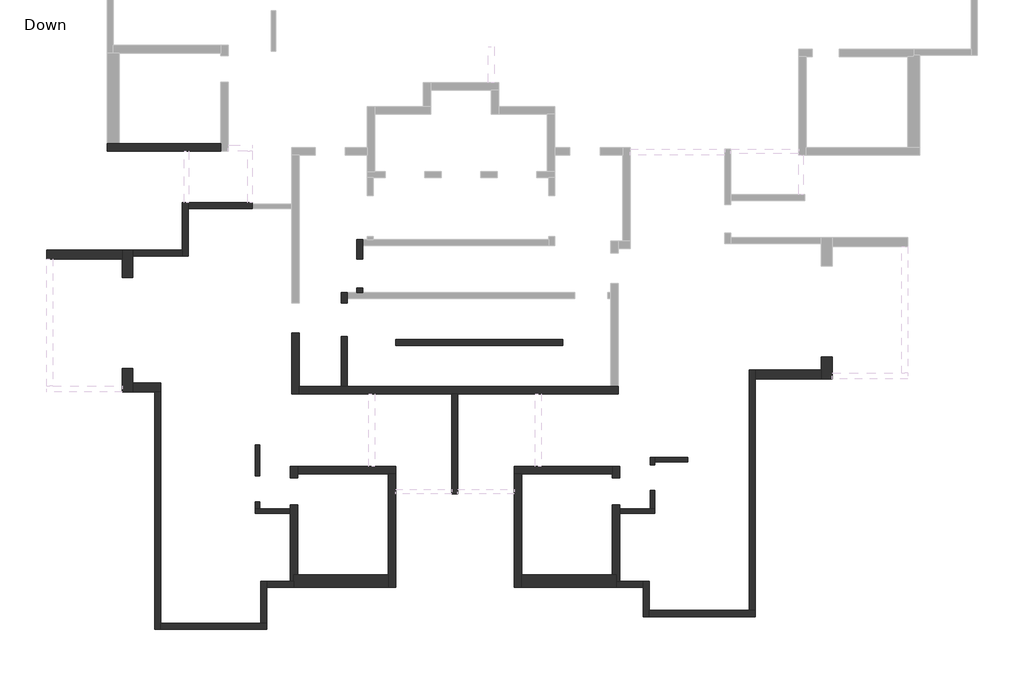
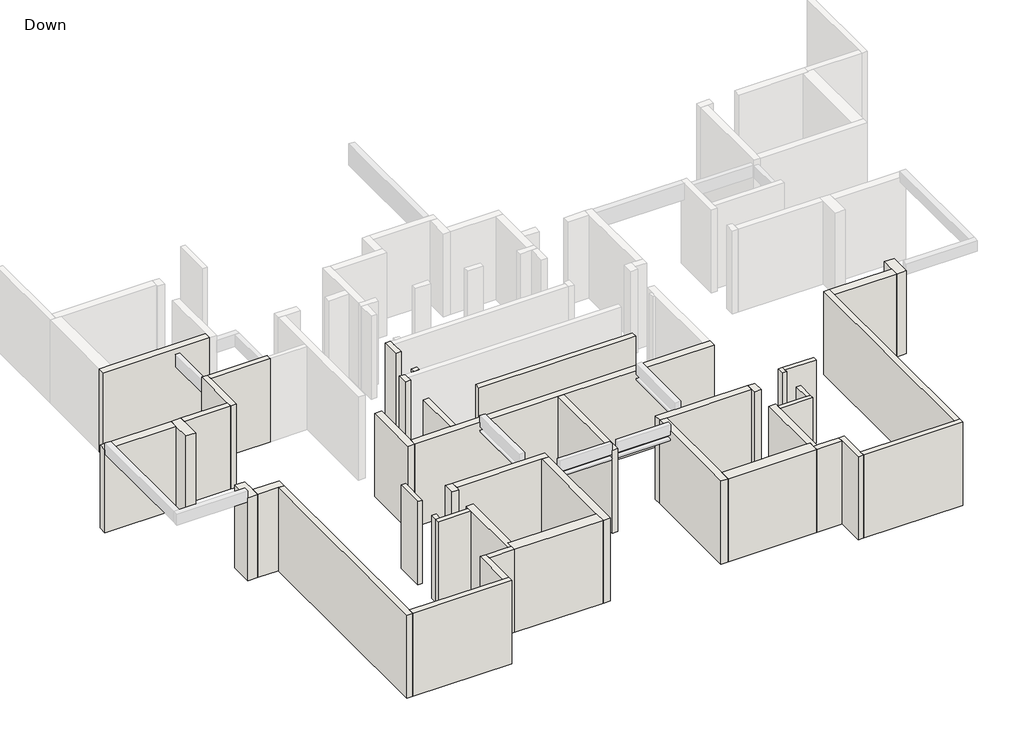
# One storey, part 1 of 3: 43 walls.
# Revit data of these elements (continued)
# Element 19 (IfcWall, "20") (continued)
#   SOFiSTiK_AMG_Adjusted = yes
#   Phase Created = New Construction
#   Base Constraint = Down
#   Top Constraint = Typical Floor
#   Materials on its faces: "Concrete"
# Element 20 (IfcWall, "20")
#   Comments = ""
#   Mark = "W36"
#   SOFiSTiK_EdgeZones = "W36"
#   SOFiSTiK_AMG_Comments = ""
#   Top Offset = 0 cm
#   Base Offset = 0 cm
#   wall height = 310 cm
#   SOFiSTiK_AMG_Scheduled = yes
#   SOFiSTiK_AMG_Adjusted = yes
#   Phase Created = New Construction
#   Base Constraint = Down
#   Top Constraint = Typical Floor
#   Materials on its faces: "Concrete"
# Element 21 (IfcWall, "20")
#   Comments = ""
#   Mark = "W37"
#   SOFiSTiK_EdgeZones = "W37"
#   SOFiSTiK_AMG_Comments = "Too Short /"
#   Top Offset = 0 cm
#   Base Offset = 0 cm
#   wall height = 310 cm
#   SOFiSTiK_AMG_Scheduled = yes
#   SOFiSTiK_AMG_Adjusted = yes
#   Phase Created = New Construction
#   Base Constraint = Down
#   Top Constraint = Typical Floor
#   Materials on its faces: "Concrete"
# Element 22 (IfcWall, "20")
#   Comments = ""
#   Mark = "W40"
#   SOFiSTiK_EdgeZones = "W40"
#   SOFiSTiK_AMG_Comments = ""
#   Top Offset = 0 cm
#   Base Offset = 0 cm
#   wall height = 310 cm
#   SOFiSTiK_AMG_Scheduled = yes
#   SOFiSTiK_AMG_Adjusted = yes
#   Phase Created = New Construction
#   Base Constraint = Down
#   Top Constraint = Typical Floor
#   Materials on its faces: "Concrete"
# Element 23 (IfcWall, "20")
#   Comments = ""
#   Mark = "W41"
#   SOFiSTiK_EdgeZones = "W41"
#   SOFiSTiK_AMG_Comments = ""
#   Top Offset = 0 cm
#   Base Offset = 0 cm
#   wall height = 310 cm
#   SOFiSTiK_AMG_Scheduled = yes
#   SOFiSTiK_AMG_Adjusted = yes
#   Phase Created = New Construction
#   Base Constraint = Down
#   Top Constraint = Typical Floor
#   Materials on its faces: "Concrete"
# Element 24 (IfcWall, "20")
#   Comments = ""
#   Mark = "W42"
#   SOFiSTiK_EdgeZones = "W42"
#   SOFiSTiK_AMG_Comments = ""
#   Top Offset = 0 cm
#   Base Offset = 0 cm
#   wall height = 310 cm
#   SOFiSTiK_AMG_Scheduled = yes
#   SOFiSTiK_AMG_Adjusted = yes
#   Phase Created = New Construction
#   Base Constraint = Down
#   Top Constraint = Typical Floor
#   Materials on its faces: "Concrete"
# Element 25 (IfcWall, "25")
#   Comments = ""
#   Mark = "W65"
#   SOFiSTiK_EdgeZones = "W65"
#   SOFiSTiK_AMG_Comments = ""
#   Top Offset = 0 cm
#   Base Offset = 0 cm
#   wall height = 310 cm
#   SOFiSTiK_AMG_Scheduled = yes
#   SOFiSTiK_AMG_Adjusted = yes
#   Phase Created = New Construction
#   Base Constraint = Down
#   Top Constraint = Typical Floor
#   Materials on its faces: "Concrete"
# Element 26 (IfcWall, "25")
#   Comments = ""
#   Mark = "W66"
#   SOFiSTiK_EdgeZones = "W66"
#   SOFiSTiK_AMG_Comments = ""
#   Top Offset = 0 cm
#   Base Offset = 0 cm
#   wall height = 310 cm
#   SOFiSTiK_AMG_Scheduled = yes
#   SOFiSTiK_AMG_Adjusted = yes
#   Phase Created = New Construction
#   Base Constraint = Down
#   Top Constraint = Typical Floor
#   Materials on its faces: "Concrete"
# Element 27 (IfcWall, "25")
#   Comments = ""
#   Mark = "W67"
#   SOFiSTiK_EdgeZones = "W67"
#   SOFiSTiK_AMG_Comments = ""
#   Top Offset = 0 cm
#   Base Offset = 0 cm
#   wall height = 310 cm
#   SOFiSTiK_AMG_Scheduled = yes
#   SOFiSTiK_AMG_Adjusted = yes
#   Phase Created = New Construction
#   Base Constraint = Down
#   Top Constraint = Typical Floor
#   Materials on its faces: "Concrete"
# Element 28 (IfcWall, "25")
#   Comments = ""
#   Mark = "W68"
#   SOFiSTiK_EdgeZones = "W68"
#   SOFiSTiK_AMG_Comments = ""
#   Top Offset = 0 cm
#   Base Offset = 0 cm
#   wall height = 310 cm
#   SOFiSTiK_AMG_Scheduled = yes
#   SOFiSTiK_AMG_Adjusted = yes
#   Phase Created = New Construction
#   Base Constraint = Down
#   Top Constraint = Typical Floor
#   Materials on its faces: "Concrete"
# Element 29 (IfcWall, "25")
#   Comments = ""
#   Mark = "W69"
#   SOFiSTiK_EdgeZones = "W69"
#   SOFiSTiK_AMG_Comments = ""
#   Top Offset = 0 cm
#   Base Offset = 0 cm
#   wall height = 310 cm
#   SOFiSTiK_AMG_Scheduled = yes
#   SOFiSTiK_AMG_Adjusted = yes
#   Phase Created = New Construction
#   Base Constraint = Down
#   Top Constraint = Typical Floor
#   Materials on its faces: "Concrete"
# Element 30 (IfcWall, "25")
#   Comments = ""
#   Mark = "W72"
#   SOFiSTiK_EdgeZones = "W72"
#   SOFiSTiK_AMG_Comments = ""
#   Top Offset = 0 cm
#   Base Offset = 0 cm
#   wall height = 310 cm
#   SOFiSTiK_AMG_Scheduled = yes
#   SOFiSTiK_AMG_Adjusted = yes
#   Phase Created = New Construction
#   Base Constraint = Down
#   Top Constraint = Typical Floor
#   Materials on its faces: "Concrete"
# Element 31 (IfcWall, "25")
#   Comments = ""
#   Mark = "W73"
#   SOFiSTiK_EdgeZones = "W73"
#   SOFiSTiK_AMG_Comments = ""
#   Top Offset = 0 cm
#   Base Offset = 0 cm
#   wall height = 310 cm
#   SOFiSTiK_AMG_Scheduled = yes
#   SOFiSTiK_AMG_Adjusted = yes
#   Phase Created = New Construction
#   Base Constraint = Down
#   Top Constraint = Typical Floor
#   Materials on its faces: "Concrete"
# Element 32 (IfcWall, "25")
#   Comments = ""
#   Mark = "W80"
#   SOFiSTiK_EdgeZones = "W84"
#   SOFiSTiK_AMG_Comments = ""
#   Top Offset = 0 cm
#   Base Offset = 0 cm
#   wall height = 310 cm
#   SOFiSTiK_AMG_Scheduled = yes
#   SOFiSTiK_AMG_Adjusted = yes
#   Phase Created = New Construction
#   Base Constraint = Down
#   Top Constraint = Typical Floor
#   Materials on its faces: "Concrete"
# Element 33 (IfcWall, "25")
#   Comments = ""
#   Mark = "W81"
#   SOFiSTiK_EdgeZones = "W85"
#   SOFiSTiK_AMG_Comments = ""
#   Top Offset = 0 cm
#   Base Offset = 0 cm
#   wall height = 310 cm
#   SOFiSTiK_AMG_Scheduled = yes
#   SOFiSTiK_AMG_Adjusted = yes
#   Phase Created = New Construction
#   Base Constraint = Down
#   Top Constraint = Typical Floor
#   Materials on its faces: "Concrete"
# Element 34 (IfcWall, "25")
#   Comments = ""
#   Mark = "W82"
#   SOFiSTiK_EdgeZones = "W86"
#   SOFiSTiK_AMG_Comments = ""
#   Top Offset = 0 cm
#   Base Offset = 0 cm
#   wall height = 310 cm
#   SOFiSTiK_AMG_Scheduled = yes
#   SOFiSTiK_AMG_Adjusted = yes
#   Phase Created = New Construction
#   Base Constraint = Down
#   Top Constraint = Typical Floor
#   Materials on its faces: "Concrete"
# Element 35 (IfcWall, "25")
#   Comments = ""
#   Mark = "W83"
#   SOFiSTiK_EdgeZones = "W87"
#   SOFiSTiK_AMG_Comments = ""
#   Top Offset = 0 cm
#   Base Offset = 0 cm
#   wall height = 310 cm
#   SOFiSTiK_AMG_Scheduled = yes
#   SOFiSTiK_AMG_Adjusted = yes
#   Phase Created = New Construction
#   Base Constraint = Down
#   Top Constraint = Typical Floor
#   Materials on its faces: "Concrete"
# Element 36 (IfcWall, "30")
#   Comments = ""
#   Mark = "W44"
#   SOFiSTiK_EdgeZones = "W44"
#   SOFiSTiK_AMG_Comments = ""
#   Top Offset = 0 cm
#   Base Offset = 0 cm
#   wall height = 310 cm
#   SOFiSTiK_AMG_Scheduled = yes
#   SOFiSTiK_AMG_Adjusted = yes
#   Phase Created = New Construction
#   Base Constraint = Down
#   Top Constraint = Typical Floor
#   Materials on its faces: "Concrete"
# Element 37 (IfcWall, "30")
#   Comments = ""
#   Mark = "W45"
#   SOFiSTiK_EdgeZones = "W45"
#   SOFiSTiK_AMG_Comments = ""
#   Top Offset = 0 cm
#   Base Offset = 0 cm
#   wall height = 310 cm
#   SOFiSTiK_AMG_Scheduled = yes
#   SOFiSTiK_AMG_Adjusted = yes
#   Phase Created = New Construction
#   Base Constraint = Down
#   Top Constraint = Typical Floor
#   Materials on its faces: "Concrete"
# Element 38 (IfcWall, "30")
#   Comments = ""
#   Mark = "W46"
#   SOFiSTiK_EdgeZones = "W46"
#   SOFiSTiK_AMG_Comments = ""
#   Top Offset = 0 cm
#   Base Offset = 0 cm
#   wall height = 310 cm
#   SOFiSTiK_AMG_Scheduled = yes
#   SOFiSTiK_AMG_Adjusted = yes
#   Phase Created = New Construction
#   Base Constraint = Down
#   Top Constraint = Typical Floor
#   Materials on its faces: "Concrete"
# Element 39 (IfcWall, "35")
#   Comments = ""
#   Mark = "W51"
#   SOFiSTiK_EdgeZones = "W51"
#   SOFiSTiK_AMG_Comments = ""
#   Top Offset = 0 cm
#   Base Offset = 0 cm
#   wall height = 310 cm
#   SOFiSTiK_AMG_Scheduled = yes
#   SOFiSTiK_AMG_Adjusted = yes
#   Phase Created = New Construction
#   Base Constraint = Down
#   Top Constraint = Typical Floor
#   Materials on its faces: "Concrete"
# Element 40 (IfcWall, "35")
#   Comments = ""
#   Mark = "W52"
#   SOFiSTiK_EdgeZones = "W52"
#   SOFiSTiK_AMG_Comments = ""
#   Top Offset = 0 cm
#   Base Offset = 0 cm
#   wall height = 310 cm
#   SOFiSTiK_AMG_Scheduled = yes
#   SOFiSTiK_AMG_Adjusted = yes
#   Phase Created = New Construction
#   Base Constraint = Down
#   Top Constraint = Typical Floor
#   Materials on its faces: "Concrete"
# Element 41 (IfcWall, "35")
#   Comments = ""
#   Mark = "W53"
#   SOFiSTiK_EdgeZones = "W53"
#   SOFiSTiK_AMG_Comments = ""
#   Top Offset = 0 cm
#   Base Offset = 0 cm
#   wall height = 310 cm
#   SOFiSTiK_AMG_Scheduled = yes
#   SOFiSTiK_AMG_Adjusted = yes
#   Phase Created = New Construction
#   Base Constraint = Down
#   Top Constraint = Typical Floor
#   Materials on its faces: "Concrete"
# Element 42 (IfcWall, "40")
#   Comments = ""
#   Mark = "W97"
#   SOFiSTiK_EdgeZones = "W101"
#   SOFiSTiK_AMG_Comments = ""
#   Top Offset = 0 cm
#   Base Offset = 0 cm
#   wall height = 310 cm
#   SOFiSTiK_AMG_Scheduled = yes
#   SOFiSTiK_AMG_Adjusted = yes
#   Phase Created = New Construction
#   Base Constraint = Down
#   Top Constraint = Typical Floor
#   Materials on its faces: "Concrete"
# Element 43 (IfcWall, "40")
#   Comments = ""
#   Mark = "W98"
#   SOFiSTiK_EdgeZones = "W102"
#   SOFiSTiK_AMG_Comments = ""
#   Top Offset = 0 cm
#   Base Offset = 0 cm
#   wall height = 310 cm
#   SOFiSTiK_AMG_Scheduled = yes
#   SOFiSTiK_AMG_Adjusted = yes
#   Phase Created = New Construction
#   Base Constraint = Down
#   Top Constraint = Typical Floor
#   Materials on its faces: "Concrete"
# Materials
#   "Concrete": class "Concrete", colour RGB 192 192 192, transparency 0, Keynote = "01000", Description = "Cast-in-place concrete", Cost = 0
